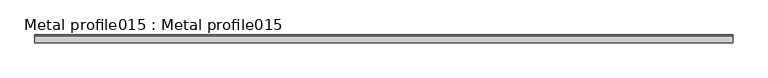
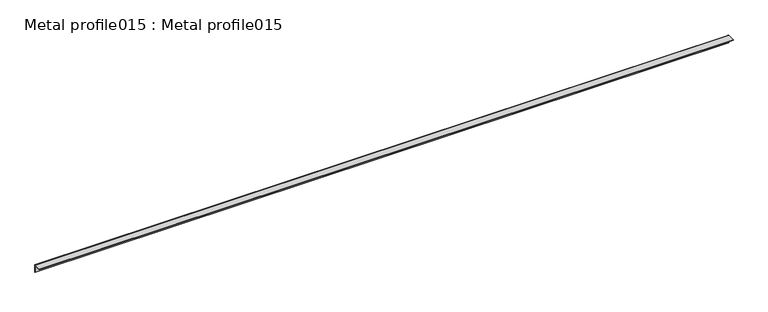
"""IFC4 building model written with IfcOpenShell, lengths in millimetres: proxy geometry, Metal profile015 : Metal profile015."""

from ifc_helpers import new_model, si_unit, point, frame, frame_2d, origin, place, context, project, spatial, polyline, circle_curve, trimmed, segment, composite_curve, outline, extrude, source, transform, mapped, element, save


def metal_profile015_metal_profile015_1b71c693(model_context):
    return source(origin(), model_context, "Body", "SweptSolid", [
        extrude(outline(composite_curve([segment(polyline([(-4258.3374811, 41076.616), (-4258.3374811, 41077.896), (-4237.4345714, 41077.896)]), True, "CONTINUOUS"), segment(trimmed(circle_curve(frame_2d((-4236.5442972, 41077.256)), 1.0964434), [point((-4237.4345714, 41077.896))], [point((-4235.9042972, 41076.3657258))], False, "CARTESIAN"), True, "CONTINUOUS"), segment(polyline([(-4235.9042972, 41076.3657258), (-4235.9042972, 41055.4628161), (-4237.1842972, 41055.4628161), (-4237.1842972, 41076.616), (-4258.3374811, 41076.616)]), True, "CONTINUOUS")], self_intersect=False)), frame((12383.0178845, 0.0, 0.0), z_axis=(1.0, 0.0, 0.0), x_axis=(0.0, 1.0, 0.0)), (0.0, 0.0, 1.0), 2000.0),
    ])


if __name__ == "__main__":
    model = new_model("IFC4")
    model_context = context("Model", 3, world=origin())
    ifc_project = project(units=[si_unit("LENGTHUNIT", "METRE", prefix="MILLI")], contexts=[model_context])
    site = spatial("IfcSite", under=ifc_project)
    building = spatial("IfcBuilding", under=site)
    placement = place(None, origin())
    metal_profile015_metal_profile015_shape = metal_profile015_metal_profile015_1b71c693(model_context)
    element("IfcBuildingElementProxy", 1, Name="Metal profile015 : Metal profile015", ObjectType="Metal profile015 : Metal profile015", at=placement, inside=building, context=model_context, shape_type="MappedRepresentation", body=[
        mapped(metal_profile015_metal_profile015_shape, transform((0.0, 0.0, 0.0), x_axis=(1.0, 0.0, 0.0), y_axis=(0.0, 1.0, 0.0), z_axis=(0.0, 0.0, 1.0))),
    ])
    save(model, "model.ifc")

# Revit data of these elements
# Type "Metal profile015 : Metal profile015"
#   NameOverride = "Metal profile015"
# Element 1 (IfcBuildingElementProxy, "Metal profile015 : Metal profile015")
#   Materials on its faces: "CORNER BEAD"
# Materials
#   "CORNER BEAD": class "Unassigned", colour RGB 253 236 176, transparency 0, Cost = 0
